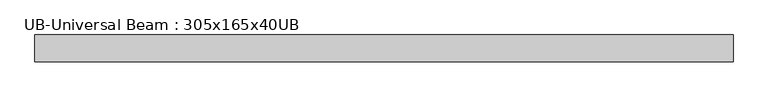
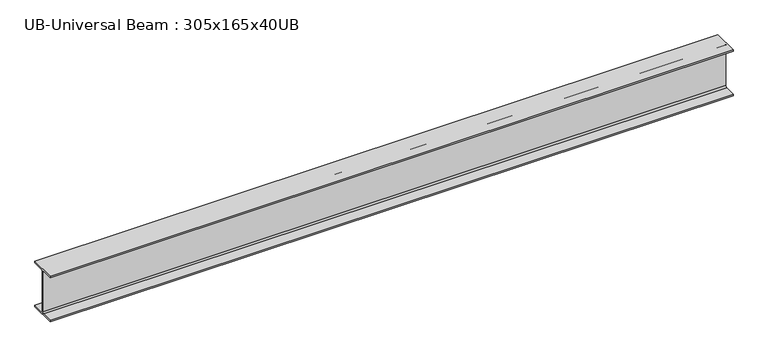
"""IFC4 building model written with IfcOpenShell, lengths in millimetres: beam geometry, UB-Universal Beam : 305x165x40UB."""

from ifc_helpers import new_model, si_unit, point, frame, frame_2d, origin, place, context, project, spatial, polyline, circle_curve, trimmed, segment, composite_curve, outline, extrude, source, transform, mapped, element, save


def ub_universal_beam_305x165x40ub_2258710d(model_context):
    return source(origin(), model_context, "Body", "SweptSolid", [
        extrude(outline(composite_curve([segment(polyline([(82.5, -141.5), (82.5, -151.7), (-82.5, -151.7), (-82.5, -141.5), (-11.9, -141.5)]), True, "CONTINUOUS"), segment(trimmed(circle_curve(frame_2d((-11.9, -132.6)), 8.9), [point((-11.9, -141.5))], [point((-3.0, -132.6))], True, "CARTESIAN"), True, "CONTINUOUS"), segment(polyline([(-3.0, -132.6), (-3.0, 132.6)]), True, "CONTINUOUS"), segment(trimmed(circle_curve(frame_2d((-11.9, 132.6)), 8.9), [point((-3.0, 132.6))], [point((-11.9, 141.5))], True, "CARTESIAN"), True, "CONTINUOUS"), segment(polyline([(-11.9, 141.5), (-82.5, 141.5), (-82.5, 151.7), (82.5, 151.7), (82.5, 141.5), (11.9, 141.5)]), True, "CONTINUOUS"), segment(trimmed(circle_curve(frame_2d((11.9, 132.6)), 8.9), [point((11.9, 141.5))], [point((3.0, 132.6))], True, "CARTESIAN"), True, "CONTINUOUS"), segment(polyline([(3.0, 132.6), (3.0, -132.6)]), True, "CONTINUOUS"), segment(trimmed(circle_curve(frame_2d((11.9, -132.6)), 8.9), [point((3.0, -132.6))], [point((11.9, -141.5))], True, "CARTESIAN"), True, "CONTINUOUS"), segment(polyline([(11.9, -141.5), (82.5, -141.5)]), True, "CONTINUOUS")], self_intersect=False)), frame((-2147.15, 0.0, 0.0), z_axis=(1.0, 0.0, 0.0), x_axis=(0.0, 1.0, 0.0)), (0.0, 0.0, 1.0), 4294.3),
    ])


if __name__ == "__main__":
    model = new_model("IFC4")
    model_context = context("Model", 3, world=origin())
    ifc_project = project(units=[si_unit("LENGTHUNIT", "METRE", prefix="MILLI")], contexts=[model_context])
    site = spatial("IfcSite", under=ifc_project)
    building = spatial("IfcBuilding", under=site)
    placement = place(None, origin())
    ub_universal_beam_305x165x40ub_shape = ub_universal_beam_305x165x40ub_2258710d(model_context)
    element("IfcBeam", 1, ObjectType="UB-Universal Beam : 305x165x40UB", at=placement, inside=building, context=model_context, shape_type="MappedRepresentation", body=[
        mapped(ub_universal_beam_305x165x40ub_shape, transform((0.0, 0.0, 0.0), x_axis=(1.0, 0.0, 0.0), y_axis=(0.0, 1.0, 0.0), z_axis=(0.0, 0.0, 1.0))),
    ])
    save(model, "model.ifc")

# Revit data of these elements
# Type "UB-Universal Beam : 305x165x40UB"
#   Nominal h = "305"
#   W = 0
#   Start Extension Calculation [instance default] = 3000 mm
#   Start Extension [instance default] = -12.7 mm
#   End Extension Calculation [instance default] = 3000 mm
#   End Extension [instance default] = -12.7 mm
#   Ix = 8503
#   Length [instance default] = 1524 mm
#   M = 40.3
#   Zx = 560
#   b = 165 mm
#   h = 303.4 mm
#   r = 8.9 mm
#   s = 6 mm
#   t = 10.2 mm
#   A = 0.005 m²
#   Structural Material [instance default] = Metal - Steel - 345 MPa
#   Assembly Code = ""
# Element 1 (IfcBeam, "UB-Universal Beam : 305x165x40UB")
#   Materials on its faces: "Metal - Steel - 345 MPa"
# Materials
#   "Metal - Steel - 345 MPa": class "Metal", colour RGB 241 46 46, transparency 0
